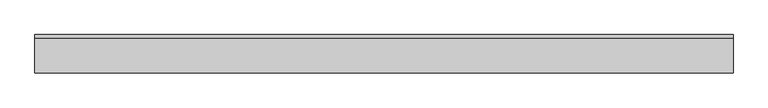
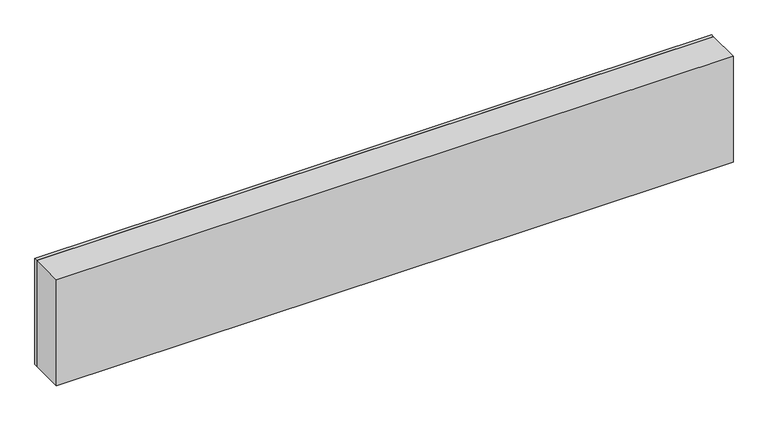
"""IFC4 building model written with IfcOpenShell, lengths in millimetres: furniture geometry, OD_CW_Upper Cabinet : OD_CW_Upper Cabinet."""

from ifc_helpers import new_model, si_unit, frame, origin, place, context, project, spatial, polyline, outline, extrude, source, transform, mapped, element, save


def furniture_9815a7d2(model_context):
    return source(origin(), model_context, "Body", "SweptSolid", [
        extrude(outline(polyline([(18.7377049, -330.2), (18.7377049, -304.8), (5543.8678379, -304.8), (5543.8678379, -330.2), (18.7377049, -330.2)])), frame((0.0, 0.0, 965.2), z_axis=(0.0, 0.0, 1.0), x_axis=(1.0, 0.0, 0.0)), (0.0, 0.0, 1.0), 914.4),
        extrude(outline(polyline([(18.7377049, -609.6), (18.7377049, -330.2), (5543.8678379, -330.2), (5543.8678379, -609.6), (18.7377049, -609.6)])), frame((0.0, 0.0, 965.2), z_axis=(0.0, 0.0, 1.0), x_axis=(1.0, 0.0, 0.0)), (0.0, 0.0, 1.0), 914.4),
    ])


if __name__ == "__main__":
    model = new_model("IFC4")
    model_context = context("Model", 3, world=origin())
    ifc_project = project(units=[si_unit("LENGTHUNIT", "METRE", prefix="MILLI")], contexts=[model_context])
    site = spatial("IfcSite", under=ifc_project)
    building = spatial("IfcBuilding", under=site)
    placement = place(None, origin())
    furniture_shape = furniture_9815a7d2(model_context)
    element("IfcFurniture", 1, ObjectType="OD_CW_Upper Cabinet : OD_CW_Upper Cabinet", at=placement, inside=building, context=model_context, shape_type="MappedRepresentation", body=[
        mapped(furniture_shape, transform((0.0, 0.0, 0.0), x_axis=(1.0, 0.0, 0.0), y_axis=(0.0, 1.0, 0.0), z_axis=(0.0, 0.0, 1.0))),
    ])
    save(model, "model.ifc")

# Revit data of these elements
# Type "OD_CW_Upper Cabinet : OD_CW_Upper Cabinet"
#   OD_CW_Width [instance default] = 2' - 2"
#   OD_CW_Off Floor [instance default] = 3' - 2"
#   OD_CW_Length [instance default] = 8' - 0"
#   OD_CW_Height [instance default] = 7' - 0"
#   Depth = 2' - 0"
#   Height = 3' - 0"
#   Width = 4' - 0"
#   OD_CW_Material_Front Panel [instance default] = none
# Element 1 (IfcFurniture, "OD_CW_Upper Cabinet : OD_CW_Upper Cabinet")
#   OD_CW_Width = 1' - 0"
#   OD_CW_Length = 18' - 1.52481"
#   OD_CW_Height = 3' - 0"
